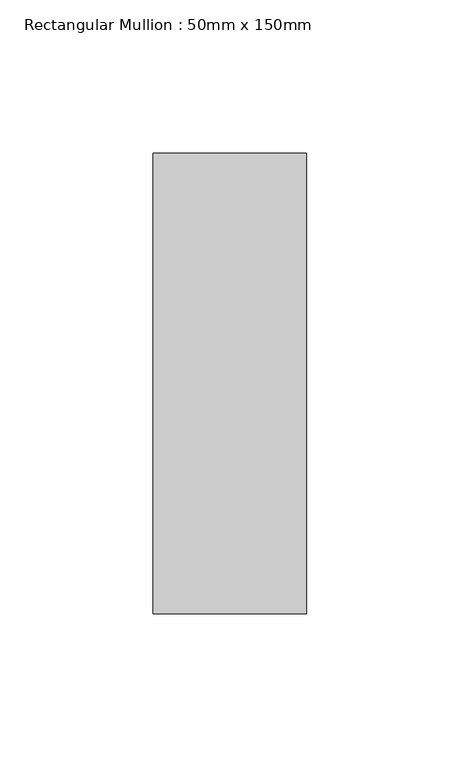
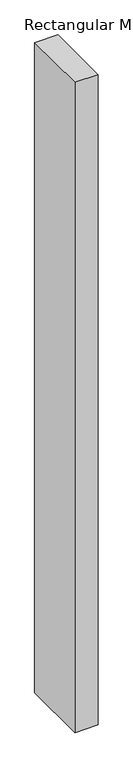
"""IFC4 building model written with IfcOpenShell, lengths in millimetres: member geometry, Rectangular Mullion : 50mm x 150mm."""

from ifc_helpers import new_model, si_unit, frame, origin, place, context, project, spatial, polyline, outline, extrude, source, transform, mapped, element, save


def rectangular_mullion_50mm_x_150mm_d77135f5(model_context):
    return source(origin(), model_context, "Body", "SweptSolid", [
        extrude(outline(polyline([(0.0, 75.0), (0.0, -75.0), (-50.0, -75.0), (-50.0, 75.0), (0.0, 75.0)])), frame((0.0, 0.0, -1484.4999997), z_axis=(0.0, 0.0, 1.0), x_axis=(1.0, 0.0, 0.0)), (0.0, 0.0, 1.0), 1484.4999997),
    ])


if __name__ == "__main__":
    model = new_model("IFC4")
    model_context = context("Model", 3, world=origin())
    ifc_project = project(units=[si_unit("LENGTHUNIT", "METRE", prefix="MILLI")], contexts=[model_context])
    site = spatial("IfcSite", under=ifc_project)
    building = spatial("IfcBuilding", under=site)
    placement = place(None, origin())
    rectangular_mullion_50mm_x_150mm_shape = rectangular_mullion_50mm_x_150mm_d77135f5(model_context)
    element("IfcMember", 1, ObjectType="Rectangular Mullion : 50mm x 150mm", at=placement, inside=building, context=model_context, shape_type="MappedRepresentation", body=[
        mapped(rectangular_mullion_50mm_x_150mm_shape, transform((0.0, 0.0, 0.0), x_axis=(1.0, 0.0, 0.0), y_axis=(0.0, 1.0, 0.0), z_axis=(0.0, 0.0, 1.0))),
    ])
    save(model, "model.ifc")

# Revit data of these elements
# Type "Rectangular Mullion : 50mm x 150mm"
#   built-in parameter 1007304 = 0.492126 (stored number, unit not read)
#   built-in parameter 1007301 = 0.082021 (stored number, unit not read)
#   built-in parameter 1007300 = 0.082021 (stored number, unit not read)
# Element 1 (IfcMember, "Rectangular Mullion : 50mm x 150mm")
#   Materials on its faces: "Aluminum"
# Materials
#   "Aluminum": class "Metal", colour RGB 244 244 244, transparency 0, Description = "Aluminum 6061", Cost = 0
